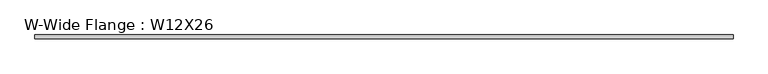
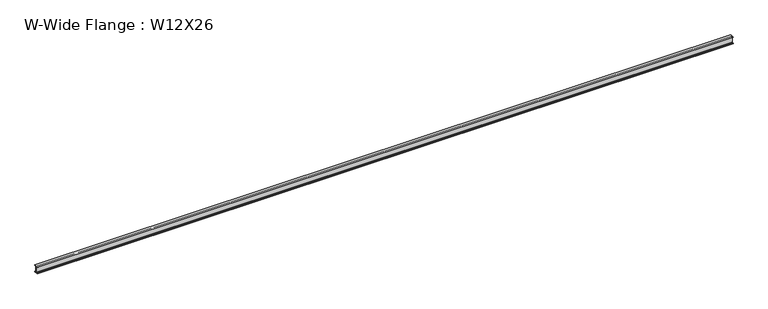
"""IFC4 building model written with IfcOpenShell, lengths in millimetres: beam geometry, W-Wide Flange : W12X26."""

from ifc_helpers import new_model, si_unit, point, frame, frame_2d, origin, place, context, project, spatial, polyline, circle_curve, trimmed, segment, composite_curve, outline, extrude, source, transform, mapped, element, save


def w_wide_flange_w12x26_eb140a27(model_context):
    return source(origin(), model_context, "Body", "SweptSolid", [
        extrude(outline(composite_curve([segment(polyline([(82.4011719, -145.5539063), (82.4011719, -155.178125), (-82.4011719, -155.178125), (-82.4011719, -145.5539063), (-20.2902344, -145.5539063)]), True, "CONTINUOUS"), segment(trimmed(circle_curve(frame_2d((-20.2902344, -128.190625)), 17.3632812), [point((-20.2902344, -145.5539063))], [point((-2.9269531, -128.190625))], True, "CARTESIAN"), True, "CONTINUOUS"), segment(polyline([(-2.9269531, -128.190625), (-2.9269531, 128.190625)]), True, "CONTINUOUS"), segment(trimmed(circle_curve(frame_2d((-20.2902344, 128.190625)), 17.3632812), [point((-2.9269531, 128.190625))], [point((-20.2902344, 145.5539062))], True, "CARTESIAN"), True, "CONTINUOUS"), segment(polyline([(-20.2902344, 145.5539062), (-82.4011719, 145.5539062), (-82.4011719, 155.178125), (82.4011719, 155.178125), (82.4011719, 145.5539062), (20.2902344, 145.5539062)]), True, "CONTINUOUS"), segment(trimmed(circle_curve(frame_2d((20.2902344, 128.190625)), 17.3632812), [point((20.2902344, 145.5539062))], [point((2.9269531, 128.190625))], True, "CARTESIAN"), True, "CONTINUOUS"), segment(polyline([(2.9269531, 128.190625), (2.9269531, -128.190625)]), True, "CONTINUOUS"), segment(trimmed(circle_curve(frame_2d((20.2902344, -128.190625)), 17.3632812), [point((2.9269531, -128.190625))], [point((20.2902344, -145.5539063))], True, "CARTESIAN"), True, "CONTINUOUS"), segment(polyline([(20.2902344, -145.5539063), (82.4011719, -145.5539063)]), True, "CONTINUOUS")], self_intersect=False)), frame((-14554.2, 0.0, 0.0), z_axis=(1.0, 0.0, 0.0), x_axis=(0.0, 1.0, 0.0)), (0.0, 0.0, 1.0), 30927.4386601),
    ])


if __name__ == "__main__":
    model = new_model("IFC4")
    model_context = context("Model", 3, world=origin())
    ifc_project = project(units=[si_unit("LENGTHUNIT", "METRE", prefix="MILLI")], contexts=[model_context])
    site = spatial("IfcSite", under=ifc_project)
    building = spatial("IfcBuilding", under=site)
    placement = place(None, origin())
    w_wide_flange_w12x26_shape = w_wide_flange_w12x26_eb140a27(model_context)
    element("IfcBeam", 1, ObjectType="W-Wide Flange : W12X26", at=placement, inside=building, context=model_context, shape_type="MappedRepresentation", body=[
        mapped(w_wide_flange_w12x26_shape, transform((0.0, 0.0, 0.0), x_axis=(1.0, 0.0, 0.0), y_axis=(0.0, 1.0, 0.0), z_axis=(0.0, 0.0, 1.0))),
    ])
    save(model, "model.ifc")

# Revit data of these elements
# Type "W-Wide Flange : W12X26"
#   Assembly Code = "B10"
#   W = 26
#   Length [instance default] = 5' - 0"
#   bf = 0' - 6 125/256"
#   d = 1' - 0 7/32"
#   k = 0' - 1 1/16"
#   k2 = 0' - 0 175/256"
#   tf = 0' - 0 97/256"
#   tw = 0' - 0 59/256"
#   A = 0.053125 SF
#   Structural Material [instance default] = none
